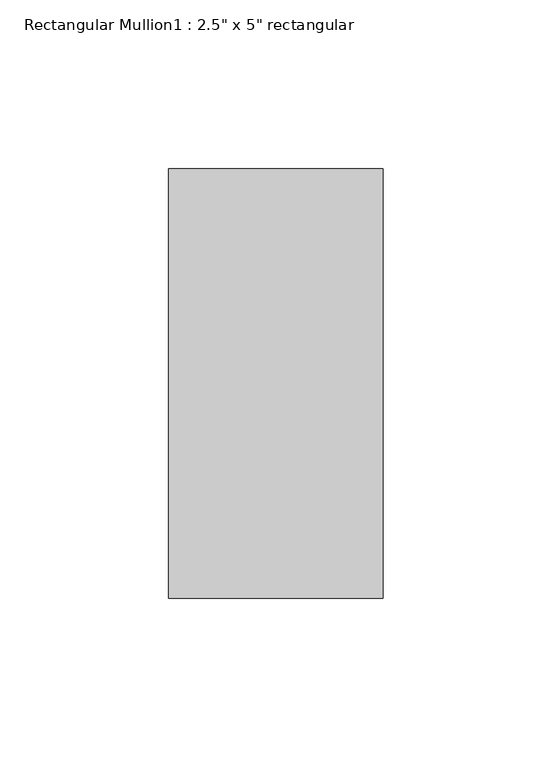
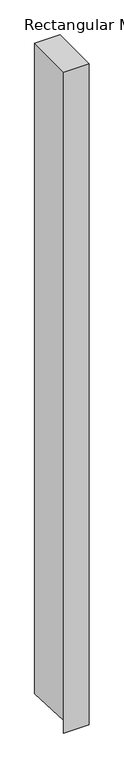
"""IFC4 building model written with IfcOpenShell, lengths in millimetres: member geometry."""

from ifc_helpers import new_model, si_unit, frame, origin, place, context, project, spatial, polyline, outline, extrude, source, transform, mapped, element, save


def member_2ed1719b(model_context):
    return source(origin(), model_context, "Body", "SweptSolid", [
        extrude(outline(polyline([(-63.5, 0.0), (63.5, 0.0), (63.5, -1736.0758182), (-62.1741259, -1731.0262636), (-63.5, -1764.0248302), (-63.5, 0.0)])), frame((-63.5, 0.0, 0.0), z_axis=(1.0, 0.0, 0.0), x_axis=(0.0, 1.0, 0.0)), (0.0, 0.0, 1.0), 63.5),
    ])


if __name__ == "__main__":
    model = new_model("IFC4")
    model_context = context("Model", 3, world=origin())
    ifc_project = project(units=[si_unit("LENGTHUNIT", "METRE", prefix="MILLI")], contexts=[model_context])
    site = spatial("IfcSite", under=ifc_project)
    building = spatial("IfcBuilding", under=site)
    placement = place(None, origin())
    member_shape = member_2ed1719b(model_context)
    element("IfcMember", 1, ObjectType="Rectangular Mullion1 : 2.5\" x 5\" rectangular", at=placement, inside=building, context=model_context, shape_type="MappedRepresentation", body=[
        mapped(member_shape, transform((0.0, 0.0, 0.0), x_axis=(1.0, 0.0, 0.0), y_axis=(0.0, 1.0, 0.0), z_axis=(0.0, 0.0, 1.0))),
    ])
    save(model, "model.ifc")

# Revit data of these elements
# Type "Rectangular Mullion1 : 2.5\" x 5\" rectangular"
#   built-in parameter 1007304 = 0.416667 (stored number, unit not read)
#   built-in parameter 1007301 = 0.104167 (stored number, unit not read)
#   built-in parameter 1007300 = 0.104167 (stored number, unit not read)
# Element 1 (IfcMember, "Rectangular Mullion1 : 2.5\" x 5\" rectangular")
#   Materials on its faces: "support-frame"
# Materials
#   "support-frame": class "Unassigned", colour RGB 233 233 233, transparency 0, Cost = 0
